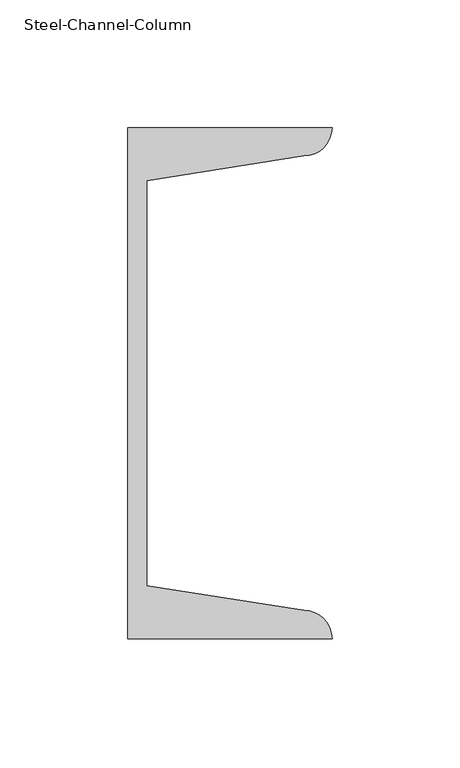
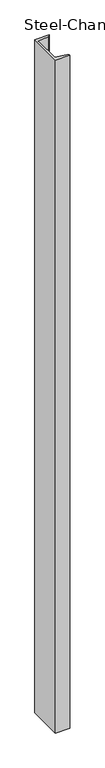
"""IFC4 building model written with IfcOpenShell, lengths in millimetres: column geometry, Steel-Channel-Column : CL126_C-200×80x7.5x11."""

import ifcopenshell
import ifcopenshell.guid

model = None  # the IFC model being written
_history = None  # IfcOwnerHistory: only IFC2X3 demands one
_inside = {}  # id of a spatial element -> (the spatial element, [elements in it])
_under = {}  # id of a project, library or spatial element -> (it, [spatial elements below it])
_declared = {}  # id of a project -> (the project, [libraries it declares])
_typed = {}  # id of a type object -> (the type object, [elements of that type])
_made_of = {}  # id of a material, layer set ... -> (it, [elements and type objects made of it])


def new_model(schema):
    """Start an empty IFC model of exactly this schema.

    Asked for "IFC4X3", IfcOpenShell would pick the latest addendum, in which some entities
    have other attributes; the version numbers below select the first issue.
    IFC2X3 requires an IfcOwnerHistory on every rooted entity: one is made here for all.
    """
    global model, _history
    if schema == "IFC4X3":
        model = ifcopenshell.file(schema_version=(4, 3, 0, 0))
    else:
        model = ifcopenshell.file(schema=schema)
    _inside.clear()
    _under.clear()
    _declared.clear()
    _typed.clear()
    _made_of.clear()
    _history = None
    if model.schema == "IFC2X3":
        org = make("IfcOrganization", Name="unknown")
        user = make(
            "IfcPersonAndOrganization",
            ThePerson=make("IfcPerson", FamilyName="unknown"),
            TheOrganization=org,
        )
        app = make(
            "IfcApplication",
            ApplicationDeveloper=org,
            Version="unknown",
            ApplicationFullName="unknown",
            ApplicationIdentifier="unknown",
        )
        _history = make(
            "IfcOwnerHistory",
            OwningUser=user,
            OwningApplication=app,
            ChangeAction="ADDED",
            CreationDate=0,
        )
    return model


def make(cls, **values):
    """One entity of the class cls with the attributes given. An attribute that is None is left unset."""
    return model.create_entity(
        cls, **{name: value for name, value in values.items() if value is not None}
    )


def rooted(cls, **values):
    """An entity with a GlobalId (a new one), such as an element, a storey or a relation."""
    return make(cls, GlobalId=ifcopenshell.guid.new(), OwnerHistory=_history, **values)


def si_unit(unit_type, name, prefix=None):
    """IfcSIUnit, for example si_unit("LENGTHUNIT", "METRE", prefix="MILLI")."""
    return make("IfcSIUnit", UnitType=unit_type, Prefix=prefix, Name=name)


def assignment(units):
    """IfcUnitAssignment: the units of a project."""
    return None if units is None else make("IfcUnitAssignment", Units=units)


def point(xyz):
    """IfcCartesianPoint."""
    return None if xyz is None else make("IfcCartesianPoint", Coordinates=xyz)


def direction(xyz):
    """IfcDirection."""
    return None if xyz is None else make("IfcDirection", DirectionRatios=xyz)


def frame(location, z_axis=None, x_axis=None):
    """IfcAxis2Placement3D, a coordinate frame: its origin and axes. An axis left out is left unset."""
    return make(
        "IfcAxis2Placement3D",
        Location=point(location),
        Axis=direction(z_axis),
        RefDirection=direction(x_axis),
    )


def frame_2d(location, x_axis=None):
    """IfcAxis2Placement2D, a coordinate frame in the plane: its origin and x axis."""
    return make(
        "IfcAxis2Placement2D", Location=point(location), RefDirection=direction(x_axis)
    )


def origin():
    """The frame at (0, 0, 0) with its axes left unset."""
    return frame((0.0, 0.0, 0.0))


def origin_with_axes():
    """The frame at (0, 0, 0) with the z axis (0, 0, 1) and the x axis (1, 0, 0) written out."""
    return frame((0.0, 0.0, 0.0), z_axis=(0.0, 0.0, 1.0), x_axis=(1.0, 0.0, 0.0))


def place(relative_to, where):
    """IfcLocalPlacement: puts the frame where relative to a parent placement (None: the world)."""
    return make(
        "IfcLocalPlacement", PlacementRelTo=relative_to, RelativePlacement=where
    )


def context(
    kind, dimensions, precision=None, world=None, true_north=None, identifier=None
):
    """IfcGeometricRepresentationContext, for example the 3D "Model" context."""
    return make(
        "IfcGeometricRepresentationContext",
        ContextIdentifier=identifier,
        ContextType=kind,
        CoordinateSpaceDimension=dimensions,
        Precision=precision,
        WorldCoordinateSystem=world,
        TrueNorth=true_north,
    )


def project(units=None, contexts=None):
    """IfcProject with its units and contexts."""
    return rooted(
        "IfcProject",
        Name="project",
        RepresentationContexts=contexts,
        UnitsInContext=assignment(units),
    )


def spatial(cls, under=None, at=None, **own):
    """A site, building, storey or space (cls), placed at a placement, below another one or the project."""
    s = rooted(cls, ObjectPlacement=at, **own)
    if under is not None:
        _under.setdefault(under.id(), (under, []))[1].append(s)
    return s


def polyline(points):
    """IfcPolyline through the points."""
    return make("IfcPolyline", Points=[point(p) for p in points])


def circle_curve(where, radius):
    """IfcCircle in the frame where."""
    return make("IfcCircle", Position=where, Radius=radius)


def trimmed(basis, trim1, trim2, sense, master):
    """IfcTrimmedCurve: the piece of a basis curve between two trims."""
    return make(
        "IfcTrimmedCurve",
        BasisCurve=basis,
        Trim1=trim1,
        Trim2=trim2,
        SenseAgreement=sense,
        MasterRepresentation=master,
    )


def segment(curve, same_sense, transition):
    """IfcCompositeCurveSegment."""
    return make(
        "IfcCompositeCurveSegment",
        Transition=transition,
        SameSense=same_sense,
        ParentCurve=curve,
    )


def composite_curve(segments, self_intersect=None):
    """IfcCompositeCurve: segments joined end to end."""
    return make("IfcCompositeCurve", Segments=segments, SelfIntersect=self_intersect)


def outline(outer, holes=None, kind="AREA"):
    """IfcArbitraryClosedProfileDef: a profile drawn as a closed curve; with holes, ...WithVoids."""
    if holes is None:
        return make("IfcArbitraryClosedProfileDef", ProfileType=kind, OuterCurve=outer)
    return make(
        "IfcArbitraryProfileDefWithVoids",
        ProfileType=kind,
        OuterCurve=outer,
        InnerCurves=holes,
    )


def extrude(swept, where, along, depth):
    """IfcExtrudedAreaSolid: the profile swept, set in the frame where, extruded along a direction by depth."""
    return make(
        "IfcExtrudedAreaSolid",
        SweptArea=swept,
        Position=where,
        ExtrudedDirection=direction(along),
        Depth=depth,
    )


def shape(context_of_items, identifier, shape_type, items):
    """IfcShapeRepresentation: the items that make up one representation, for example the "Body"."""
    return make(
        "IfcShapeRepresentation",
        ContextOfItems=context_of_items,
        RepresentationIdentifier=identifier,
        RepresentationType=shape_type,
        Items=items,
    )


def source(mapping_origin, context_of_items, identifier, shape_type, items):
    """IfcRepresentationMap: a shape defined once, which mapped items show again and again."""
    return make(
        "IfcRepresentationMap",
        MappingOrigin=mapping_origin,
        MappedRepresentation=shape(context_of_items, identifier, shape_type, items),
    )


def transform(
    local_origin,
    x_axis=None,
    y_axis=None,
    z_axis=None,
    scale=None,
    scale2=None,
    scale3=None,
    uniform=True,
):
    """IfcCartesianTransformationOperator3D, or its non-uniform kind. x_axis, y_axis, z_axis: its Axis1, 2, 3."""
    if uniform:
        return make(
            "IfcCartesianTransformationOperator3D",
            Axis1=direction(x_axis),
            Axis2=direction(y_axis),
            LocalOrigin=point(local_origin),
            Scale=scale,
            Axis3=direction(z_axis),
        )
    return make(
        "IfcCartesianTransformationOperator3DnonUniform",
        Axis1=direction(x_axis),
        Axis2=direction(y_axis),
        LocalOrigin=point(local_origin),
        Scale=scale,
        Axis3=direction(z_axis),
        Scale2=scale2,
        Scale3=scale3,
    )


def mapped(mapping_source, mapping_target):
    """IfcMappedItem: shows the shape of a source again, moved by a transform."""
    return make(
        "IfcMappedItem", MappingSource=mapping_source, MappingTarget=mapping_target
    )


def made_of(thing, what):
    """Note that an element or type object is made of a material, layer set ...; save() writes the relation."""
    if what is not None:
        _made_of.setdefault(what.id(), (what, []))[1].append(thing)
    return thing


def element(
    cls,
    number,
    at=None,
    inside=None,
    cuts=None,
    type_object=None,
    material=None,
    context=None,
    identifier="Body",
    shape_type=None,
    held_by="IfcProductDefinitionShape",
    body=None,
    shapes=None,
    **own,
):
    """One element of the class cls, such as IfcWall. Its Tag is "e" and its number.

    at: its placement. inside: the storey or other place that contains it. cuts: it is an
    opening in that element (IfcRelVoidsElement). A single representation is given by context,
    identifier, shape_type and body (its items); several are given by shapes. held_by: the class
    of the entity that holds the representations. save() writes the other relations.
    """
    e = rooted(cls, Tag="e%d" % number, ObjectPlacement=at, **own)
    if body is not None:
        shapes = [shape(context, identifier, shape_type, body)]
    if shapes is not None:
        e.Representation = make(held_by, Representations=shapes)
    if inside is not None:
        _inside.setdefault(inside.id(), (inside, []))[1].append(e)
    if cuts is not None:
        rooted(
            "IfcRelVoidsElement", RelatingBuildingElement=cuts, RelatedOpeningElement=e
        )
    if type_object is not None:
        _typed.setdefault(type_object.id(), (type_object, []))[1].append(e)
    return made_of(e, material)


def aggregate(whole, parts):
    """IfcRelAggregates: a whole, such as a stair, and the parts it consists of."""
    return rooted("IfcRelAggregates", RelatingObject=whole, RelatedObjects=parts)


def save(model, path):
    """Write the relations noted so far, then the file.

    IfcRelAggregates (storeys below a building ...), IfcRelContainedInSpatialStructure (elements
    in a storey), IfcRelDefinesByType, IfcRelAssociatesMaterial and IfcRelDeclares: one each for
    every whole, place, type object, material and project.
    """
    for whole, parts in _under.values():
        aggregate(whole, parts)
    for where, things in _inside.values():
        rooted(
            "IfcRelContainedInSpatialStructure",
            RelatedElements=things,
            RelatingStructure=where,
        )
    for kind, things in _typed.values():
        rooted("IfcRelDefinesByType", RelatedObjects=things, RelatingType=kind)
    for what, things in _made_of.values():
        rooted("IfcRelAssociatesMaterial", RelatedObjects=things, RelatingMaterial=what)
    for by, libraries in _declared.values():
        rooted("IfcRelDeclares", RelatingContext=by, RelatedDefinitions=libraries)
    model.write(path)


def steel_channel_column_727a91eb(model_context):
    return source(origin(), model_context, "Body", "SweptSolid", [
        extrude(outline(composite_curve([segment(polyline([(-22.1, -100.0), (-22.1, 100.0), (57.9, 100.0)]), True, "CONTINUOUS"), segment(trimmed(circle_curve(frame_2d((46.9, 100.0)), 11.0), [point((57.9, 100.0))], [point((46.9, 89.0))], False, "CARTESIAN"), True, "CONTINUOUS"), segment(polyline([(46.9, 89.0), (-14.6, 79.2593569), (-14.6, -79.2593569), (46.9, -89.0)]), True, "CONTINUOUS"), segment(trimmed(circle_curve(frame_2d((46.9, -100.0)), 11.0), [point((46.9, -89.0))], [point((57.9, -100.0))], False, "CARTESIAN"), True, "CONTINUOUS"), segment(polyline([(57.9, -100.0), (-22.1, -100.0)]), True, "CONTINUOUS")], self_intersect=False)), origin_with_axes(), (0.0, 0.0, 1.0), 4000.0),
    ])


if __name__ == "__main__":
    model = new_model("IFC4")
    model_context = context("Model", 3, world=origin())
    ifc_project = project(units=[si_unit("LENGTHUNIT", "METRE", prefix="MILLI")], contexts=[model_context])
    site = spatial("IfcSite", under=ifc_project)
    building = spatial("IfcBuilding", under=site)
    placement = place(None, origin())
    steel_channel_column_shape = steel_channel_column_727a91eb(model_context)
    element("IfcColumn", 1, ObjectType="Steel-Channel-Column : CL126_C-200×80x7.5x11", at=placement, inside=building, context=model_context, shape_type="MappedRepresentation", body=[
        mapped(steel_channel_column_shape, transform((0.0, 0.0, 0.0), x_axis=(1.0, 0.0, 0.0), y_axis=(0.0, 1.0, 0.0), z_axis=(0.0, 0.0, 1.0))),
    ])
    save(model, "model.ifc")

# Revit data of these elements
# Type "Steel-Channel-Column : CL126_C-200×80x7.5x11"
#   Assembly Code = "B10"
#   x = 22.1 mm
#   Section Area = 31.33 cm²
#   Mass per Unit Length = 24.60 kg/m
#   bf = 80 mm
#   d = 200 mm
#   tf = 11 mm
#   tw = 7.5 mm
#   hec_material4 [instance default] = none
#   hec_material3 [instance default] = none
#   hec_material2 [instance default] = none
#   hec_material1 [instance default] = none
#   Structural Material [instance default] = Steel, 45-345
# Element 1 (IfcColumn, "Steel-Channel-Column : CL126_C-200×80x7.5x11")
#   Materials on its faces: "Steel, 45-345"
# Materials
#   "Steel, 45-345": class "Metal", colour RGB 189 187 185, transparency 0, Description = "Steel 345 MPa", Cost = 0
